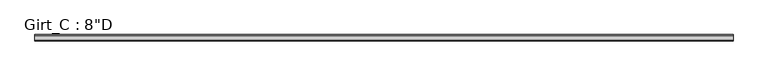
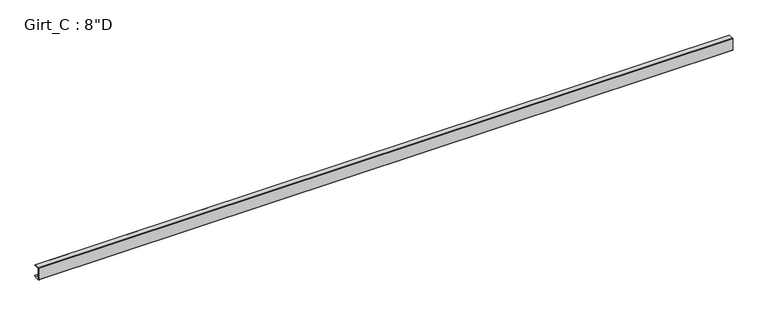
"""IFC4 building model written with IfcOpenShell, lengths in millimetres: beam geometry."""

from ifc_helpers import new_model, si_unit, point, frame, frame_2d, origin, place, context, project, spatial, polyline, circle_curve, trimmed, segment, composite_curve, outline, extrude, source, transform, mapped, element, save


def beam_bbeaa923(model_context):
    return source(origin(), model_context, "Body", "SweptSolid", [
        extrude(outline(composite_curve([segment(polyline([(87.5109375, 101.6), (99.7560415, 87.0068534), (97.6278742, 85.221109), (86.2154765, 98.821875), (3.3005807, 98.821875)]), True, "CONTINUOUS"), segment(trimmed(circle_curve(frame_2d((3.3741066, 96.8381931)), 1.9850441), [point((3.3005807, 98.821875))], [point((1.3890625, 96.8381931))], True, "CARTESIAN"), True, "CONTINUOUS"), segment(polyline([(1.3890625, 96.8381931), (1.3890625, -96.8389339)]), True, "CONTINUOUS"), segment(trimmed(circle_curve(frame_2d((3.3748024, -96.8389339)), 1.9857399), [point((1.3890625, -96.8389339))], [point((3.2694106, -98.821875))], True, "CARTESIAN"), True, "CONTINUOUS"), segment(polyline([(3.2694106, -98.821875), (86.2154765, -98.821875), (97.6510975, -85.1934327), (99.7792647, -86.979177), (87.5109375, -101.6), (3.3734375, -101.6)]), True, "CONTINUOUS"), segment(trimmed(circle_curve(frame_2d((3.3734375, -96.8375)), 4.7625), [point((3.3734375, -101.6))], [point((-1.3890625, -96.8375))], False, "CARTESIAN"), True, "CONTINUOUS"), segment(polyline([(-1.3890625, -96.8375), (-1.3890625, 96.8375)]), True, "CONTINUOUS"), segment(trimmed(circle_curve(frame_2d((3.3734375, 96.8375)), 4.7625), [point((-1.3890625, 96.8375))], [point((3.3734375, 101.6))], False, "CARTESIAN"), True, "CONTINUOUS"), segment(polyline([(3.3734375, 101.6), (87.5109375, 101.6)]), True, "CONTINUOUS")], self_intersect=False)), frame((-5611.449741, 0.0, 0.0), z_axis=(1.0, 0.0, 0.0), x_axis=(0.0, 1.0, 0.0)), (0.0, 0.0, 1.0), 11245.419389),
    ])


if __name__ == "__main__":
    model = new_model("IFC4")
    model_context = context("Model", 3, world=origin())
    ifc_project = project(units=[si_unit("LENGTHUNIT", "METRE", prefix="MILLI")], contexts=[model_context])
    site = spatial("IfcSite", under=ifc_project)
    building = spatial("IfcBuilding", under=site)
    placement = place(None, origin())
    beam_shape = beam_bbeaa923(model_context)
    element("IfcBeam", 1, ObjectType="Girt_C : 8\"D", at=placement, inside=building, context=model_context, shape_type="MappedRepresentation", body=[
        mapped(beam_shape, transform((0.0, 0.0, 0.0), x_axis=(1.0, 0.0, 0.0), y_axis=(0.0, 1.0, 0.0), z_axis=(0.0, 0.0, 1.0))),
    ])
    save(model, "model.ifc")

# Revit data of these elements
# Type "Girt_C : 8\"D"
#   half leg = 0' - 1 3/4"
#   Web_Thickness = 0' - 0 7/64"
#   Length [instance default] = 10' - 0"
#   Leg_1 = 0' - 3 1/2"
#   Height = 0' - 8"
#   Structural Material [instance default] = none
# Element 1 (IfcBeam, "Girt_C : 8\"D")
#   Structural Material = CEE' SECTION (8.0x3.5C - SEE STRUCT. DWGS)
#   Materials on its faces: "CEE' SECTION (8.0x3.5C - SEE STRUCT. DWGS)"
# Materials
#   "CEE' SECTION (8.0x3.5C - SEE STRUCT. DWGS)": class "Metal", colour RGB 137 146 153, transparency 0, Description = "Steel, mill finish", Cost = 0
